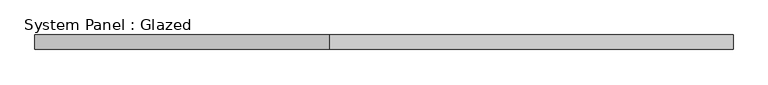
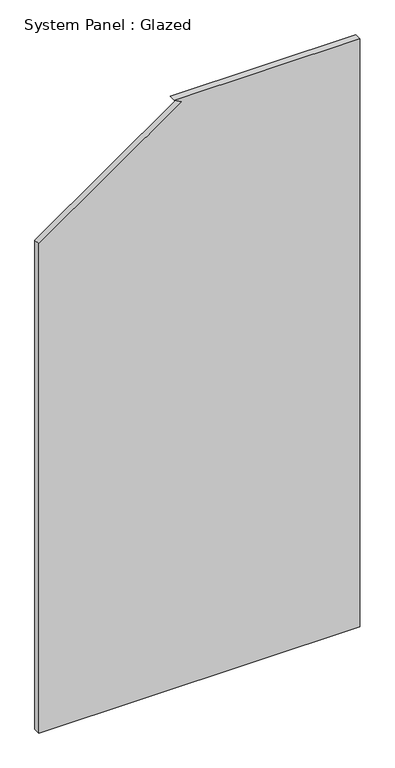
"""IFC4 building model written with IfcOpenShell, lengths in millimetres: plate geometry, System Panel : Glazed."""

import ifcopenshell
import ifcopenshell.guid

model = None  # the IFC model being written
_history = None  # IfcOwnerHistory: only IFC2X3 demands one
_inside = {}  # id of a spatial element -> (the spatial element, [elements in it])
_under = {}  # id of a project, library or spatial element -> (it, [spatial elements below it])
_declared = {}  # id of a project -> (the project, [libraries it declares])
_typed = {}  # id of a type object -> (the type object, [elements of that type])
_made_of = {}  # id of a material, layer set ... -> (it, [elements and type objects made of it])


def new_model(schema):
    """Start an empty IFC model of exactly this schema.

    Asked for "IFC4X3", IfcOpenShell would pick the latest addendum, in which some entities
    have other attributes; the version numbers below select the first issue.
    IFC2X3 requires an IfcOwnerHistory on every rooted entity: one is made here for all.
    """
    global model, _history
    if schema == "IFC4X3":
        model = ifcopenshell.file(schema_version=(4, 3, 0, 0))
    else:
        model = ifcopenshell.file(schema=schema)
    _inside.clear()
    _under.clear()
    _declared.clear()
    _typed.clear()
    _made_of.clear()
    _history = None
    if model.schema == "IFC2X3":
        org = make("IfcOrganization", Name="unknown")
        user = make(
            "IfcPersonAndOrganization",
            ThePerson=make("IfcPerson", FamilyName="unknown"),
            TheOrganization=org,
        )
        app = make(
            "IfcApplication",
            ApplicationDeveloper=org,
            Version="unknown",
            ApplicationFullName="unknown",
            ApplicationIdentifier="unknown",
        )
        _history = make(
            "IfcOwnerHistory",
            OwningUser=user,
            OwningApplication=app,
            ChangeAction="ADDED",
            CreationDate=0,
        )
    return model


def make(cls, **values):
    """One entity of the class cls with the attributes given. An attribute that is None is left unset."""
    return model.create_entity(
        cls, **{name: value for name, value in values.items() if value is not None}
    )


def rooted(cls, **values):
    """An entity with a GlobalId (a new one), such as an element, a storey or a relation."""
    return make(cls, GlobalId=ifcopenshell.guid.new(), OwnerHistory=_history, **values)


def si_unit(unit_type, name, prefix=None):
    """IfcSIUnit, for example si_unit("LENGTHUNIT", "METRE", prefix="MILLI")."""
    return make("IfcSIUnit", UnitType=unit_type, Prefix=prefix, Name=name)


def assignment(units):
    """IfcUnitAssignment: the units of a project."""
    return None if units is None else make("IfcUnitAssignment", Units=units)


def point(xyz):
    """IfcCartesianPoint."""
    return None if xyz is None else make("IfcCartesianPoint", Coordinates=xyz)


def direction(xyz):
    """IfcDirection."""
    return None if xyz is None else make("IfcDirection", DirectionRatios=xyz)


def frame(location, z_axis=None, x_axis=None):
    """IfcAxis2Placement3D, a coordinate frame: its origin and axes. An axis left out is left unset."""
    return make(
        "IfcAxis2Placement3D",
        Location=point(location),
        Axis=direction(z_axis),
        RefDirection=direction(x_axis),
    )


def origin():
    """The frame at (0, 0, 0) with its axes left unset."""
    return frame((0.0, 0.0, 0.0))


def place(relative_to, where):
    """IfcLocalPlacement: puts the frame where relative to a parent placement (None: the world)."""
    return make(
        "IfcLocalPlacement", PlacementRelTo=relative_to, RelativePlacement=where
    )


def context(
    kind, dimensions, precision=None, world=None, true_north=None, identifier=None
):
    """IfcGeometricRepresentationContext, for example the 3D "Model" context."""
    return make(
        "IfcGeometricRepresentationContext",
        ContextIdentifier=identifier,
        ContextType=kind,
        CoordinateSpaceDimension=dimensions,
        Precision=precision,
        WorldCoordinateSystem=world,
        TrueNorth=true_north,
    )


def project(units=None, contexts=None):
    """IfcProject with its units and contexts."""
    return rooted(
        "IfcProject",
        Name="project",
        RepresentationContexts=contexts,
        UnitsInContext=assignment(units),
    )


def spatial(cls, under=None, at=None, **own):
    """A site, building, storey or space (cls), placed at a placement, below another one or the project."""
    s = rooted(cls, ObjectPlacement=at, **own)
    if under is not None:
        _under.setdefault(under.id(), (under, []))[1].append(s)
    return s


def polyline(points):
    """IfcPolyline through the points."""
    return make("IfcPolyline", Points=[point(p) for p in points])


def outline(outer, holes=None, kind="AREA"):
    """IfcArbitraryClosedProfileDef: a profile drawn as a closed curve; with holes, ...WithVoids."""
    if holes is None:
        return make("IfcArbitraryClosedProfileDef", ProfileType=kind, OuterCurve=outer)
    return make(
        "IfcArbitraryProfileDefWithVoids",
        ProfileType=kind,
        OuterCurve=outer,
        InnerCurves=holes,
    )


def extrude(swept, where, along, depth):
    """IfcExtrudedAreaSolid: the profile swept, set in the frame where, extruded along a direction by depth."""
    return make(
        "IfcExtrudedAreaSolid",
        SweptArea=swept,
        Position=where,
        ExtrudedDirection=direction(along),
        Depth=depth,
    )


def shape(context_of_items, identifier, shape_type, items):
    """IfcShapeRepresentation: the items that make up one representation, for example the "Body"."""
    return make(
        "IfcShapeRepresentation",
        ContextOfItems=context_of_items,
        RepresentationIdentifier=identifier,
        RepresentationType=shape_type,
        Items=items,
    )


def source(mapping_origin, context_of_items, identifier, shape_type, items):
    """IfcRepresentationMap: a shape defined once, which mapped items show again and again."""
    return make(
        "IfcRepresentationMap",
        MappingOrigin=mapping_origin,
        MappedRepresentation=shape(context_of_items, identifier, shape_type, items),
    )


def transform(
    local_origin,
    x_axis=None,
    y_axis=None,
    z_axis=None,
    scale=None,
    scale2=None,
    scale3=None,
    uniform=True,
):
    """IfcCartesianTransformationOperator3D, or its non-uniform kind. x_axis, y_axis, z_axis: its Axis1, 2, 3."""
    if uniform:
        return make(
            "IfcCartesianTransformationOperator3D",
            Axis1=direction(x_axis),
            Axis2=direction(y_axis),
            LocalOrigin=point(local_origin),
            Scale=scale,
            Axis3=direction(z_axis),
        )
    return make(
        "IfcCartesianTransformationOperator3DnonUniform",
        Axis1=direction(x_axis),
        Axis2=direction(y_axis),
        LocalOrigin=point(local_origin),
        Scale=scale,
        Axis3=direction(z_axis),
        Scale2=scale2,
        Scale3=scale3,
    )


def mapped(mapping_source, mapping_target):
    """IfcMappedItem: shows the shape of a source again, moved by a transform."""
    return make(
        "IfcMappedItem", MappingSource=mapping_source, MappingTarget=mapping_target
    )


def made_of(thing, what):
    """Note that an element or type object is made of a material, layer set ...; save() writes the relation."""
    if what is not None:
        _made_of.setdefault(what.id(), (what, []))[1].append(thing)
    return thing


def element(
    cls,
    number,
    at=None,
    inside=None,
    cuts=None,
    type_object=None,
    material=None,
    context=None,
    identifier="Body",
    shape_type=None,
    held_by="IfcProductDefinitionShape",
    body=None,
    shapes=None,
    **own,
):
    """One element of the class cls, such as IfcWall. Its Tag is "e" and its number.

    at: its placement. inside: the storey or other place that contains it. cuts: it is an
    opening in that element (IfcRelVoidsElement). A single representation is given by context,
    identifier, shape_type and body (its items); several are given by shapes. held_by: the class
    of the entity that holds the representations. save() writes the other relations.
    """
    e = rooted(cls, Tag="e%d" % number, ObjectPlacement=at, **own)
    if body is not None:
        shapes = [shape(context, identifier, shape_type, body)]
    if shapes is not None:
        e.Representation = make(held_by, Representations=shapes)
    if inside is not None:
        _inside.setdefault(inside.id(), (inside, []))[1].append(e)
    if cuts is not None:
        rooted(
            "IfcRelVoidsElement", RelatingBuildingElement=cuts, RelatedOpeningElement=e
        )
    if type_object is not None:
        _typed.setdefault(type_object.id(), (type_object, []))[1].append(e)
    return made_of(e, material)


def aggregate(whole, parts):
    """IfcRelAggregates: a whole, such as a stair, and the parts it consists of."""
    return rooted("IfcRelAggregates", RelatingObject=whole, RelatedObjects=parts)


def save(model, path):
    """Write the relations noted so far, then the file.

    IfcRelAggregates (storeys below a building ...), IfcRelContainedInSpatialStructure (elements
    in a storey), IfcRelDefinesByType, IfcRelAssociatesMaterial and IfcRelDeclares: one each for
    every whole, place, type object, material and project.
    """
    for whole, parts in _under.values():
        aggregate(whole, parts)
    for where, things in _inside.values():
        rooted(
            "IfcRelContainedInSpatialStructure",
            RelatedElements=things,
            RelatingStructure=where,
        )
    for kind, things in _typed.values():
        rooted("IfcRelDefinesByType", RelatedObjects=things, RelatingType=kind)
    for what, things in _made_of.values():
        rooted("IfcRelAssociatesMaterial", RelatedObjects=things, RelatingMaterial=what)
    for by, libraries in _declared.values():
        rooted("IfcRelDeclares", RelatingContext=by, RelatedDefinitions=libraries)
    model.write(path)


def system_panel_glazed_7f2b43f2(model_context):
    return source(origin(), model_context, "Body", "SweptSolid", [
        extrude(outline(polyline([(0.0, -600.0), (0.0, 600.0), (2325.0, 600.0), (2325.0, -93.111196), (2309.0423978, -64.4323741), (1934.0339089, -600.0), (0.0, -600.0)])), frame((0.0, -49.5, 0.0), z_axis=(0.0, 1.0, 0.0), x_axis=(0.0, 0.0, 1.0)), (0.0, 0.0, 1.0), 25.0),
    ])


if __name__ == "__main__":
    model = new_model("IFC4")
    model_context = context("Model", 3, world=origin())
    ifc_project = project(units=[si_unit("LENGTHUNIT", "METRE", prefix="MILLI")], contexts=[model_context])
    site = spatial("IfcSite", under=ifc_project)
    building = spatial("IfcBuilding", under=site)
    placement = place(None, origin())
    system_panel_glazed_shape = system_panel_glazed_7f2b43f2(model_context)
    element("IfcPlate", 1, ObjectType="System Panel : Glazed", at=placement, inside=building, context=model_context, shape_type="MappedRepresentation", body=[
        mapped(system_panel_glazed_shape, transform((0.0, 0.0, 0.0), x_axis=(1.0, 0.0, 0.0), y_axis=(0.0, 1.0, 0.0), z_axis=(0.0, 0.0, 1.0))),
    ])
    save(model, "model.ifc")

# Revit data of these elements
# Type "System Panel : Glazed"
#   Construction Type Id = "GSP4R"
#   Analytic Construction = "1/8 in Pilkington single glazing"
#   Visual Light Transmittance = 0.9
#   Solar Heat Gain Coefficient = 0.86
#   Heat Transfer Coefficient (U) = 6.7069 W/(m²·K)
#   Define Thermal Properties by = 1
# Element 1 (IfcPlate, "System Panel : Glazed")
#   Materials on its faces: "Glass"
# Materials
#   "Glass": class "Glass", colour RGB 0 128 192, transparency 0.9, Description = "Soda Lime Glass", Cost = 0
